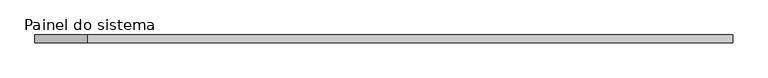
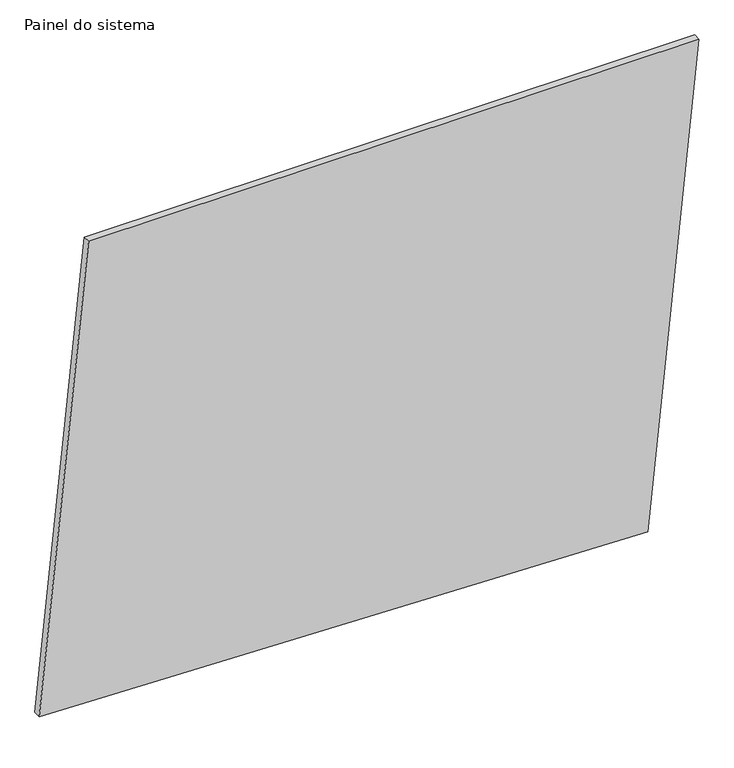
"""IFC4 building model written with IfcOpenShell, lengths in millimetres: plate geometry, Painel do sistema : Envidraçado."""

import ifcopenshell
import ifcopenshell.guid

model = None  # the IFC model being written
_history = None  # IfcOwnerHistory: only IFC2X3 demands one
_inside = {}  # id of a spatial element -> (the spatial element, [elements in it])
_under = {}  # id of a project, library or spatial element -> (it, [spatial elements below it])
_declared = {}  # id of a project -> (the project, [libraries it declares])
_typed = {}  # id of a type object -> (the type object, [elements of that type])
_made_of = {}  # id of a material, layer set ... -> (it, [elements and type objects made of it])


def new_model(schema):
    """Start an empty IFC model of exactly this schema.

    Asked for "IFC4X3", IfcOpenShell would pick the latest addendum, in which some entities
    have other attributes; the version numbers below select the first issue.
    IFC2X3 requires an IfcOwnerHistory on every rooted entity: one is made here for all.
    """
    global model, _history
    if schema == "IFC4X3":
        model = ifcopenshell.file(schema_version=(4, 3, 0, 0))
    else:
        model = ifcopenshell.file(schema=schema)
    _inside.clear()
    _under.clear()
    _declared.clear()
    _typed.clear()
    _made_of.clear()
    _history = None
    if model.schema == "IFC2X3":
        org = make("IfcOrganization", Name="unknown")
        user = make(
            "IfcPersonAndOrganization",
            ThePerson=make("IfcPerson", FamilyName="unknown"),
            TheOrganization=org,
        )
        app = make(
            "IfcApplication",
            ApplicationDeveloper=org,
            Version="unknown",
            ApplicationFullName="unknown",
            ApplicationIdentifier="unknown",
        )
        _history = make(
            "IfcOwnerHistory",
            OwningUser=user,
            OwningApplication=app,
            ChangeAction="ADDED",
            CreationDate=0,
        )
    return model


def make(cls, **values):
    """One entity of the class cls with the attributes given. An attribute that is None is left unset."""
    return model.create_entity(
        cls, **{name: value for name, value in values.items() if value is not None}
    )


def rooted(cls, **values):
    """An entity with a GlobalId (a new one), such as an element, a storey or a relation."""
    return make(cls, GlobalId=ifcopenshell.guid.new(), OwnerHistory=_history, **values)


def si_unit(unit_type, name, prefix=None):
    """IfcSIUnit, for example si_unit("LENGTHUNIT", "METRE", prefix="MILLI")."""
    return make("IfcSIUnit", UnitType=unit_type, Prefix=prefix, Name=name)


def assignment(units):
    """IfcUnitAssignment: the units of a project."""
    return None if units is None else make("IfcUnitAssignment", Units=units)


def point(xyz):
    """IfcCartesianPoint."""
    return None if xyz is None else make("IfcCartesianPoint", Coordinates=xyz)


def direction(xyz):
    """IfcDirection."""
    return None if xyz is None else make("IfcDirection", DirectionRatios=xyz)


def frame(location, z_axis=None, x_axis=None):
    """IfcAxis2Placement3D, a coordinate frame: its origin and axes. An axis left out is left unset."""
    return make(
        "IfcAxis2Placement3D",
        Location=point(location),
        Axis=direction(z_axis),
        RefDirection=direction(x_axis),
    )


def origin():
    """The frame at (0, 0, 0) with its axes left unset."""
    return frame((0.0, 0.0, 0.0))


def place(relative_to, where):
    """IfcLocalPlacement: puts the frame where relative to a parent placement (None: the world)."""
    return make(
        "IfcLocalPlacement", PlacementRelTo=relative_to, RelativePlacement=where
    )


def context(
    kind, dimensions, precision=None, world=None, true_north=None, identifier=None
):
    """IfcGeometricRepresentationContext, for example the 3D "Model" context."""
    return make(
        "IfcGeometricRepresentationContext",
        ContextIdentifier=identifier,
        ContextType=kind,
        CoordinateSpaceDimension=dimensions,
        Precision=precision,
        WorldCoordinateSystem=world,
        TrueNorth=true_north,
    )


def project(units=None, contexts=None):
    """IfcProject with its units and contexts."""
    return rooted(
        "IfcProject",
        Name="project",
        RepresentationContexts=contexts,
        UnitsInContext=assignment(units),
    )


def spatial(cls, under=None, at=None, **own):
    """A site, building, storey or space (cls), placed at a placement, below another one or the project."""
    s = rooted(cls, ObjectPlacement=at, **own)
    if under is not None:
        _under.setdefault(under.id(), (under, []))[1].append(s)
    return s


def polyline(points):
    """IfcPolyline through the points."""
    return make("IfcPolyline", Points=[point(p) for p in points])


def outline(outer, holes=None, kind="AREA"):
    """IfcArbitraryClosedProfileDef: a profile drawn as a closed curve; with holes, ...WithVoids."""
    if holes is None:
        return make("IfcArbitraryClosedProfileDef", ProfileType=kind, OuterCurve=outer)
    return make(
        "IfcArbitraryProfileDefWithVoids",
        ProfileType=kind,
        OuterCurve=outer,
        InnerCurves=holes,
    )


def extrude(swept, where, along, depth):
    """IfcExtrudedAreaSolid: the profile swept, set in the frame where, extruded along a direction by depth."""
    return make(
        "IfcExtrudedAreaSolid",
        SweptArea=swept,
        Position=where,
        ExtrudedDirection=direction(along),
        Depth=depth,
    )


def shape(context_of_items, identifier, shape_type, items):
    """IfcShapeRepresentation: the items that make up one representation, for example the "Body"."""
    return make(
        "IfcShapeRepresentation",
        ContextOfItems=context_of_items,
        RepresentationIdentifier=identifier,
        RepresentationType=shape_type,
        Items=items,
    )


def source(mapping_origin, context_of_items, identifier, shape_type, items):
    """IfcRepresentationMap: a shape defined once, which mapped items show again and again."""
    return make(
        "IfcRepresentationMap",
        MappingOrigin=mapping_origin,
        MappedRepresentation=shape(context_of_items, identifier, shape_type, items),
    )


def transform(
    local_origin,
    x_axis=None,
    y_axis=None,
    z_axis=None,
    scale=None,
    scale2=None,
    scale3=None,
    uniform=True,
):
    """IfcCartesianTransformationOperator3D, or its non-uniform kind. x_axis, y_axis, z_axis: its Axis1, 2, 3."""
    if uniform:
        return make(
            "IfcCartesianTransformationOperator3D",
            Axis1=direction(x_axis),
            Axis2=direction(y_axis),
            LocalOrigin=point(local_origin),
            Scale=scale,
            Axis3=direction(z_axis),
        )
    return make(
        "IfcCartesianTransformationOperator3DnonUniform",
        Axis1=direction(x_axis),
        Axis2=direction(y_axis),
        LocalOrigin=point(local_origin),
        Scale=scale,
        Axis3=direction(z_axis),
        Scale2=scale2,
        Scale3=scale3,
    )


def mapped(mapping_source, mapping_target):
    """IfcMappedItem: shows the shape of a source again, moved by a transform."""
    return make(
        "IfcMappedItem", MappingSource=mapping_source, MappingTarget=mapping_target
    )


def made_of(thing, what):
    """Note that an element or type object is made of a material, layer set ...; save() writes the relation."""
    if what is not None:
        _made_of.setdefault(what.id(), (what, []))[1].append(thing)
    return thing


def element(
    cls,
    number,
    at=None,
    inside=None,
    cuts=None,
    type_object=None,
    material=None,
    context=None,
    identifier="Body",
    shape_type=None,
    held_by="IfcProductDefinitionShape",
    body=None,
    shapes=None,
    **own,
):
    """One element of the class cls, such as IfcWall. Its Tag is "e" and its number.

    at: its placement. inside: the storey or other place that contains it. cuts: it is an
    opening in that element (IfcRelVoidsElement). A single representation is given by context,
    identifier, shape_type and body (its items); several are given by shapes. held_by: the class
    of the entity that holds the representations. save() writes the other relations.
    """
    e = rooted(cls, Tag="e%d" % number, ObjectPlacement=at, **own)
    if body is not None:
        shapes = [shape(context, identifier, shape_type, body)]
    if shapes is not None:
        e.Representation = make(held_by, Representations=shapes)
    if inside is not None:
        _inside.setdefault(inside.id(), (inside, []))[1].append(e)
    if cuts is not None:
        rooted(
            "IfcRelVoidsElement", RelatingBuildingElement=cuts, RelatedOpeningElement=e
        )
    if type_object is not None:
        _typed.setdefault(type_object.id(), (type_object, []))[1].append(e)
    return made_of(e, material)


def aggregate(whole, parts):
    """IfcRelAggregates: a whole, such as a stair, and the parts it consists of."""
    return rooted("IfcRelAggregates", RelatingObject=whole, RelatedObjects=parts)


def save(model, path):
    """Write the relations noted so far, then the file.

    IfcRelAggregates (storeys below a building ...), IfcRelContainedInSpatialStructure (elements
    in a storey), IfcRelDefinesByType, IfcRelAssociatesMaterial and IfcRelDeclares: one each for
    every whole, place, type object, material and project.
    """
    for whole, parts in _under.values():
        aggregate(whole, parts)
    for where, things in _inside.values():
        rooted(
            "IfcRelContainedInSpatialStructure",
            RelatedElements=things,
            RelatingStructure=where,
        )
    for kind, things in _typed.values():
        rooted("IfcRelDefinesByType", RelatedObjects=things, RelatingType=kind)
    for what, things in _made_of.values():
        rooted("IfcRelAssociatesMaterial", RelatedObjects=things, RelatingMaterial=what)
    for by, libraries in _declared.values():
        rooted("IfcRelDeclares", RelatingContext=by, RelatedDefinitions=libraries)
    model.write(path)


def painel_do_sistema_b016b202(model_context):
    return source(origin(), model_context, "Body", "SweptSolid", [
        extrude(outline(polyline([(59.2714287, -1120.0284238), (0.0, 946.4380919), (1706.4612154, 1120.0284238), (1706.4612154, -952.4674976), (59.2714287, -1120.0284238)])), frame((0.0, 24.5, 0.0), z_axis=(0.0, 1.0, 0.0), x_axis=(0.0, 0.0, 1.0)), (0.0, 0.0, 1.0), 25.0),
    ])


if __name__ == "__main__":
    model = new_model("IFC4")
    model_context = context("Model", 3, world=origin())
    ifc_project = project(units=[si_unit("LENGTHUNIT", "METRE", prefix="MILLI")], contexts=[model_context])
    site = spatial("IfcSite", under=ifc_project)
    building = spatial("IfcBuilding", under=site)
    placement = place(None, origin())
    painel_do_sistema_shape = painel_do_sistema_b016b202(model_context)
    element("IfcPlate", 1, ObjectType="Painel do sistema : Envidraçado", at=placement, inside=building, context=model_context, shape_type="MappedRepresentation", body=[
        mapped(painel_do_sistema_shape, transform((0.0, 0.0, 0.0), x_axis=(1.0, 0.0, 0.0), y_axis=(0.0, 1.0, 0.0), z_axis=(0.0, 0.0, 1.0))),
    ])
    save(model, "model.ifc")

# Revit data of these elements
# Type "Painel do sistema : Envidraçado"
#   Construction Type Id = "GSP4R"
#   Analytic Construction = "Vidraça única Pilkington 1/8 pol"
#   Visual Light Transmittance = 0.9
#   Solar Heat Gain Coefficient = 0.86
#   Heat Transfer Coefficient (U) = 6.7069 W/(m²·K)
# Element 1 (IfcPlate, "Painel do sistema : Envidraçado")
#   Materials on its faces: "Vidro"
# Materials
#   "Vidro": class "Vidro", colour RGB 0 128 192, transparency 0.9, Description = "Vidro de sílica", Cost = 0
